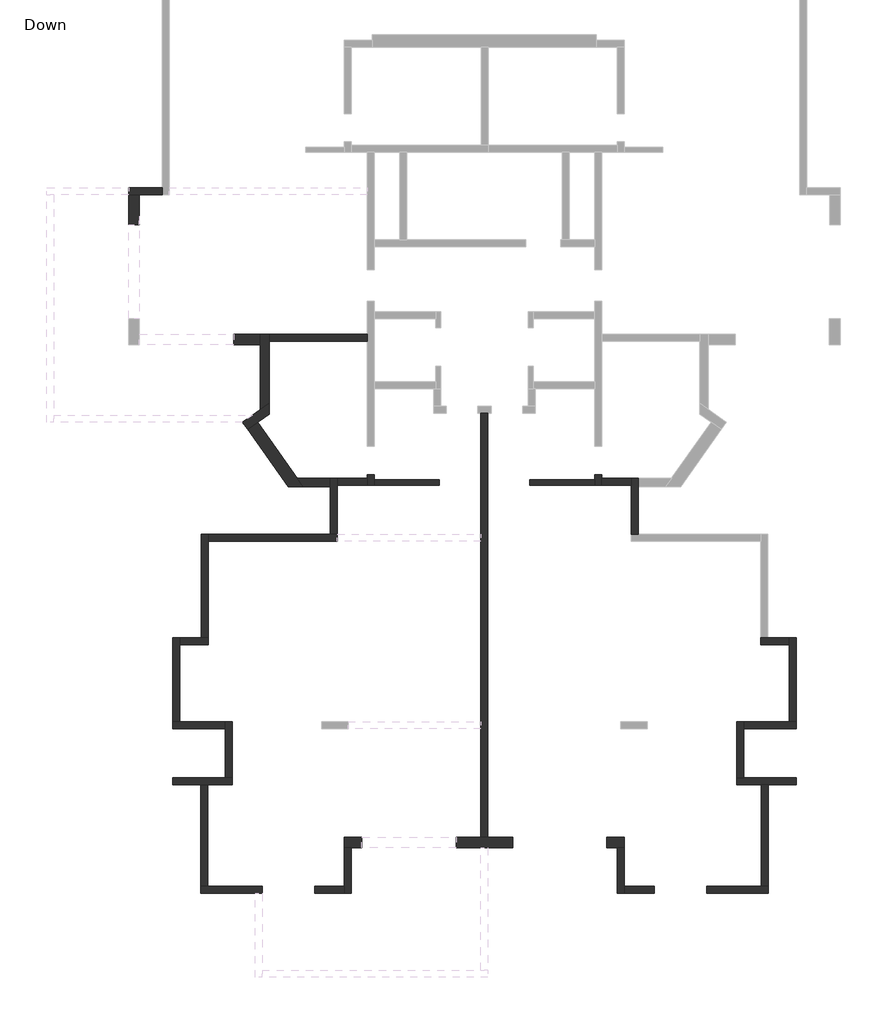
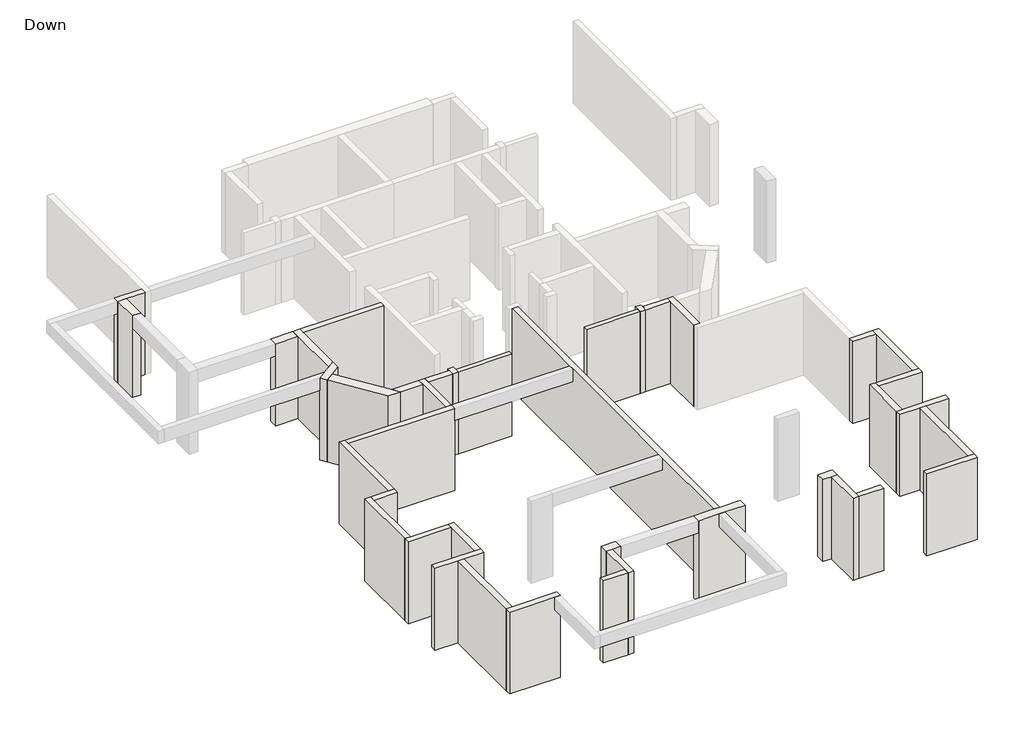
# One storey, part 1 of 3: 40 walls.
"""IFC4 building model written with IfcOpenShell, lengths in millimetres."""

import ifcopenshell
import ifcopenshell.guid

model = None  # the IFC model being written
_history = None  # IfcOwnerHistory: only IFC2X3 demands one
_inside = {}  # id of a spatial element -> (the spatial element, [elements in it])
_under = {}  # id of a project, library or spatial element -> (it, [spatial elements below it])
_declared = {}  # id of a project -> (the project, [libraries it declares])
_typed = {}  # id of a type object -> (the type object, [elements of that type])
_made_of = {}  # id of a material, layer set ... -> (it, [elements and type objects made of it])


def new_model(schema):
    """Start an empty IFC model of exactly this schema.

    Asked for "IFC4X3", IfcOpenShell would pick the latest addendum, in which some entities
    have other attributes; the version numbers below select the first issue.
    IFC2X3 requires an IfcOwnerHistory on every rooted entity: one is made here for all.
    """
    global model, _history
    if schema == "IFC4X3":
        model = ifcopenshell.file(schema_version=(4, 3, 0, 0))
    else:
        model = ifcopenshell.file(schema=schema)
    _inside.clear()
    _under.clear()
    _declared.clear()
    _typed.clear()
    _made_of.clear()
    _history = None
    if model.schema == "IFC2X3":
        org = make("IfcOrganization", Name="unknown")
        user = make(
            "IfcPersonAndOrganization",
            ThePerson=make("IfcPerson", FamilyName="unknown"),
            TheOrganization=org,
        )
        app = make(
            "IfcApplication",
            ApplicationDeveloper=org,
            Version="unknown",
            ApplicationFullName="unknown",
            ApplicationIdentifier="unknown",
        )
        _history = make(
            "IfcOwnerHistory",
            OwningUser=user,
            OwningApplication=app,
            ChangeAction="ADDED",
            CreationDate=0,
        )
    return model


def make(cls, **values):
    """One entity of the class cls with the attributes given. An attribute that is None is left unset."""
    return model.create_entity(
        cls, **{name: value for name, value in values.items() if value is not None}
    )


def rooted(cls, **values):
    """An entity with a GlobalId (a new one), such as an element, a storey or a relation."""
    return make(cls, GlobalId=ifcopenshell.guid.new(), OwnerHistory=_history, **values)


def si_unit(unit_type, name, prefix=None):
    """IfcSIUnit, for example si_unit("LENGTHUNIT", "METRE", prefix="MILLI")."""
    return make("IfcSIUnit", UnitType=unit_type, Prefix=prefix, Name=name)


def assignment(units):
    """IfcUnitAssignment: the units of a project."""
    return None if units is None else make("IfcUnitAssignment", Units=units)


def point(xyz):
    """IfcCartesianPoint."""
    return None if xyz is None else make("IfcCartesianPoint", Coordinates=xyz)


def direction(xyz):
    """IfcDirection."""
    return None if xyz is None else make("IfcDirection", DirectionRatios=xyz)


def frame(location, z_axis=None, x_axis=None):
    """IfcAxis2Placement3D, a coordinate frame: its origin and axes. An axis left out is left unset."""
    return make(
        "IfcAxis2Placement3D",
        Location=point(location),
        Axis=direction(z_axis),
        RefDirection=direction(x_axis),
    )


def origin():
    """The frame at (0, 0, 0) with its axes left unset."""
    return frame((0.0, 0.0, 0.0))


def place(relative_to, where):
    """IfcLocalPlacement: puts the frame where relative to a parent placement (None: the world)."""
    return make(
        "IfcLocalPlacement", PlacementRelTo=relative_to, RelativePlacement=where
    )


def context(
    kind, dimensions, precision=None, world=None, true_north=None, identifier=None
):
    """IfcGeometricRepresentationContext, for example the 3D "Model" context."""
    return make(
        "IfcGeometricRepresentationContext",
        ContextIdentifier=identifier,
        ContextType=kind,
        CoordinateSpaceDimension=dimensions,
        Precision=precision,
        WorldCoordinateSystem=world,
        TrueNorth=true_north,
    )


def project(units=None, contexts=None):
    """IfcProject with its units and contexts."""
    return rooted(
        "IfcProject",
        Name="project",
        RepresentationContexts=contexts,
        UnitsInContext=assignment(units),
    )


def spatial(cls, under=None, at=None, **own):
    """A site, building, storey or space (cls), placed at a placement, below another one or the project."""
    s = rooted(cls, ObjectPlacement=at, **own)
    if under is not None:
        _under.setdefault(under.id(), (under, []))[1].append(s)
    return s


def faces_of(points, faces, orient=None, outer=None):
    """IfcFace entities. A face is a list of loops; a loop is a list of indices into points, from 0.

    orient and outer hold one flag for each loop. By default every Orientation is true, the
    first loop of a face is its IfcFaceOuterBound and the others are IfcFaceBound.
    """
    made = []
    for i, loops in enumerate(faces):
        bounds = []
        for j, loop in enumerate(loops):
            is_outer = j == 0 if outer is None else outer[i][j]
            bounds.append(
                make(
                    "IfcFaceOuterBound" if is_outer else "IfcFaceBound",
                    Bound=make("IfcPolyLoop", Polygon=[points[k] for k in loop]),
                    Orientation=True if orient is None else orient[i][j],
                )
            )
        made.append(make("IfcFace", Bounds=bounds))
    return made


def faceted_brep(points, faces, orient=None, outer=None, voids=None):
    """IfcFacetedBrep: a solid bounded by flat faces; with voids (closed shells), ...WithVoids."""
    shared = [point(p) for p in points]
    hull = make("IfcClosedShell", CfsFaces=faces_of(shared, faces, orient, outer))
    if voids is None:
        return make("IfcFacetedBrep", Outer=hull)
    return make(
        "IfcFacetedBrepWithVoids",
        Outer=hull,
        Voids=[
            make(cls, CfsFaces=faces_of(shared, fs, o, b)) for cls, fs, o, b in voids
        ],
    )


def shape(context_of_items, identifier, shape_type, items):
    """IfcShapeRepresentation: the items that make up one representation, for example the "Body"."""
    return make(
        "IfcShapeRepresentation",
        ContextOfItems=context_of_items,
        RepresentationIdentifier=identifier,
        RepresentationType=shape_type,
        Items=items,
    )


def made_of(thing, what):
    """Note that an element or type object is made of a material, layer set ...; save() writes the relation."""
    if what is not None:
        _made_of.setdefault(what.id(), (what, []))[1].append(thing)
    return thing


def element(
    cls,
    number,
    at=None,
    inside=None,
    cuts=None,
    type_object=None,
    material=None,
    context=None,
    identifier="Body",
    shape_type=None,
    held_by="IfcProductDefinitionShape",
    body=None,
    shapes=None,
    **own,
):
    """One element of the class cls, such as IfcWall. Its Tag is "e" and its number.

    at: its placement. inside: the storey or other place that contains it. cuts: it is an
    opening in that element (IfcRelVoidsElement). A single representation is given by context,
    identifier, shape_type and body (its items); several are given by shapes. held_by: the class
    of the entity that holds the representations. save() writes the other relations.
    """
    e = rooted(cls, Tag="e%d" % number, ObjectPlacement=at, **own)
    if body is not None:
        shapes = [shape(context, identifier, shape_type, body)]
    if shapes is not None:
        e.Representation = make(held_by, Representations=shapes)
    if inside is not None:
        _inside.setdefault(inside.id(), (inside, []))[1].append(e)
    if cuts is not None:
        rooted(
            "IfcRelVoidsElement", RelatingBuildingElement=cuts, RelatedOpeningElement=e
        )
    if type_object is not None:
        _typed.setdefault(type_object.id(), (type_object, []))[1].append(e)
    return made_of(e, material)


def aggregate(whole, parts):
    """IfcRelAggregates: a whole, such as a stair, and the parts it consists of."""
    return rooted("IfcRelAggregates", RelatingObject=whole, RelatedObjects=parts)


def save(model, path):
    """Write the relations noted so far, then the file.

    IfcRelAggregates (storeys below a building ...), IfcRelContainedInSpatialStructure (elements
    in a storey), IfcRelDefinesByType, IfcRelAssociatesMaterial and IfcRelDeclares: one each for
    every whole, place, type object, material and project.
    """
    for whole, parts in _under.values():
        aggregate(whole, parts)
    for where, things in _inside.values():
        rooted(
            "IfcRelContainedInSpatialStructure",
            RelatedElements=things,
            RelatingStructure=where,
        )
    for kind, things in _typed.values():
        rooted("IfcRelDefinesByType", RelatedObjects=things, RelatingType=kind)
    for what, things in _made_of.values():
        rooted("IfcRelAssociatesMaterial", RelatedObjects=things, RelatingMaterial=what)
    for by, libraries in _declared.values():
        rooted("IfcRelDeclares", RelatingContext=by, RelatedDefinitions=libraries)
    model.write(path)


model = new_model("IFC4")

# Units and contexts
model_context = context("Model", 3, world=origin())
ifc_project = project(units=[si_unit("LENGTHUNIT", "METRE", prefix="MILLI")], contexts=[model_context])

# Site, building, storey
site = spatial("IfcSite", under=ifc_project)
building = spatial("IfcBuilding", under=site)
storey = spatial("IfcBuildingStorey", under=building, Name="Down", Elevation=0.0)

# Walls
placement = place(None, origin())
element("IfcWall", 1, ObjectType="15", at=placement, inside=storey, context=model_context, shape_type="Brep", body=[
    faceted_brep([(877.2376347, -8447.6409767, 0.0), (2726.9065089, -8447.6409767, 0.0), (2726.9065089, -8447.6409767, 2800.0), (2726.9065089, -8447.6409767, 3000.0), (877.2376347, -8447.6409767, 3000.0), (877.2376347, -8297.6409767, 0.0), (877.2376347, -8297.6409767, 2800.0), (877.2376347, -8297.6409767, 3000.0), (2726.9065089, -8297.6409767, 3000.0), (2726.9065089, -8297.6409767, 2800.0), (2726.9065089, -8297.6409767, 0.0)], [[[0, 1, 2, 3, 4]], [[5, 6, 7, 8, 9, 10]], [[1, 0, 5, 10]], [[3, 2, 1, 10, 9, 8]], [[4, 3, 8, 7]], [[0, 4, 7, 6, 5]]]),
])
element("IfcWall", 2, ObjectType="15", at=placement, inside=storey, context=model_context, shape_type="Brep", body=[
    faceted_brep([(7169.9528665, -8297.6409767, 0.0), (5320.2839923, -8297.6409767, 0.0), (5320.2839923, -8297.6409767, 2800.0), (5320.2839923, -8297.6409767, 3000.0), (7169.9528665, -8297.6409767, 3000.0), (7169.9528665, -8297.6409767, 2800.0), (7169.9528665, -8447.6409767, 0.0), (7169.9528665, -8447.6409767, 3000.0), (5320.2839923, -8447.6409767, 3000.0), (5320.2839923, -8447.6409767, 2800.0), (5320.2839923, -8447.6409767, 0.0)], [[[0, 1, 2, 3, 4, 5]], [[6, 7, 8, 9, 10]], [[1, 0, 6, 10]], [[3, 2, 1, 10, 9, 8]], [[4, 3, 8, 7]], [[0, 5, 4, 7, 6]]]),
])
element("IfcWall", 3, ObjectType="20", at=placement, inside=storey, context=model_context, shape_type="Brep", body=[
    faceted_brep([(-5177.0670011, 46.6636591, 0.0), (-6127.9594861, 46.6636591, 0.0), (-6127.9594861, 46.6636591, 2550.0), (-6127.9594861, 46.6636591, 3000.0), (-5177.0670011, 46.6636591, 3000.0), (-5177.0670011, -153.3363409, 0.0), (-5177.0670011, -153.3363409, 3000.0), (-5827.9594861, -153.3363409, 3000.0), (-6127.9594861, -153.3363409, 3000.0), (-6127.9594861, -153.3363409, 2550.0), (-6127.9594861, -153.3363409, 0.0), (-5827.9594861, -153.3363409, 0.0)], [[[0, 1, 2, 3, 4]], [[5, 6, 7, 8, 9, 10, 11]], [[1, 0, 5, 11, 10]], [[4, 3, 8, 7, 6]], [[0, 4, 6, 5]], [[3, 2, 1, 10, 9, 8]]]),
])
element("IfcWall", 4, ObjectType="20", at=placement, inside=storey, context=model_context, shape_type="Brep", body=[
    faceted_brep([(3923.5952506, -6391.6807118, 0.0), (3923.5952506, -18496.3164734, 0.0), (3923.5952506, -18496.3164734, 2800.0), (3923.5952506, -18496.3164734, 3000.0), (3923.5952506, -15399.2157792, 3000.0), (3923.5952506, -15199.2157792, 3000.0), (3923.5952506, -10045.6542217, 3000.0), (3923.5952506, -9845.6542217, 3000.0), (3923.5952506, -6391.6807118, 3000.0), (3923.5952506, -6391.6807118, 2800.0), (4123.5952506, -6391.6807118, 0.0), (4123.5952506, -6391.6807118, 2800.0), (4123.5952506, -6391.6807118, 3000.0), (4123.5952506, -9845.6542217, 3000.0), (4123.5952506, -10045.6542217, 3000.0), (4123.5952506, -15199.2157792, 3000.0), (4123.5952506, -15399.2157792, 3000.0), (4123.5952506, -18496.3164734, 3000.0), (4123.5952506, -18496.3164734, 2800.0), (4123.5952506, -18496.3164734, 0.0)], [[[0, 1, 2, 3, 4, 5, 6, 7, 8, 9]], [[10, 11, 12, 13, 14, 15, 16, 17, 18, 19]], [[1, 0, 10, 19]], [[8, 7, 6, 5, 4, 3, 17, 16, 15, 14, 13, 12]], [[0, 9, 8, 12, 11, 10]], [[3, 2, 1, 19, 18, 17]]]),
])
element("IfcWall", 5, ObjectType="20", at=placement, inside=storey, context=model_context, shape_type="Brep", body=[
    faceted_brep([(27.8998864, -18796.3164734, 0.0), (27.8998864, -19900.6211091, 0.0), (27.8998864, -20100.6211091, 0.0), (27.8998864, -20100.6211091, 3000.0), (27.8998864, -19900.6211091, 3000.0), (27.8998864, -18796.3164734, 3000.0), (227.8998864, -18796.3164734, 0.0), (227.8998864, -18796.3164734, 2800.0), (227.8998864, -18796.3164734, 3000.0), (227.8998864, -20100.6211091, 3000.0), (227.8998864, -20100.6211091, 2800.0), (227.8998864, -20100.6211091, 0.0)], [[[0, 1, 2, 3, 4, 5]], [[6, 7, 8, 9, 10, 11]], [[2, 1, 0, 6, 11]], [[5, 4, 3, 9, 8]], [[0, 5, 8, 7, 6]], [[3, 2, 11, 10, 9]]]),
])
element("IfcWall", 6, ObjectType="20", at=placement, inside=storey, context=model_context, shape_type="Brep", body=[
    faceted_brep([(27.8998864, -19900.6211091, 0.0), (-827.7292527, -19900.6211091, 0.0), (-827.7292527, -19900.6211091, 2800.0), (-827.7292527, -19900.6211091, 3000.0), (27.8998864, -19900.6211091, 3000.0), (27.8998864, -19900.6211091, 2800.0), (27.8998864, -20100.6211091, 0.0), (27.8998864, -20100.6211091, 3000.0), (-827.7292527, -20100.6211091, 3000.0), (-827.7292527, -20100.6211091, 2800.0), (-827.7292527, -20100.6211091, 0.0)], [[[0, 1, 2, 3, 4, 5]], [[6, 7, 8, 9, 10]], [[1, 0, 6, 10]], [[3, 2, 1, 10, 9, 8]], [[4, 3, 8, 7]], [[0, 5, 4, 7, 6]]]),
])
element("IfcWall", 7, ObjectType="20", at=placement, inside=storey, context=model_context, shape_type="Brep", body=[
    faceted_brep([(-2325.0802461, -19900.6211091, 0.0), (-3874.0868686, -19900.6211091, 0.0), (-4074.0868686, -19900.6211091, 0.0), (-4074.0868686, -19900.6211091, 3000.0), (-3874.0868686, -19900.6211091, 3000.0), (-2325.0802461, -19900.6211091, 3000.0), (-2325.0802461, -19900.6211091, 2800.0), (-2325.0802461, -20100.6211091, 0.0), (-2325.0802461, -20100.6211091, 2800.0), (-2325.0802461, -20100.6211091, 3000.0), (-4074.0868686, -20100.6211091, 3000.0), (-4074.0868686, -20100.6211091, 0.0)], [[[0, 1, 2, 3, 4, 5, 6]], [[7, 8, 9, 10, 11]], [[2, 1, 0, 7, 11]], [[5, 4, 3, 10, 9]], [[0, 6, 5, 9, 8, 7]], [[3, 2, 11, 10]]]),
])
element("IfcWall", 8, ObjectType="20", at=placement, inside=storey, context=model_context, shape_type="Brep", body=[
    faceted_brep([(-3874.0868686, -19900.6211091, 0.0), (-3874.0868686, -16998.96548, 0.0), (-3874.0868686, -16998.96548, 2800.0), (-3874.0868686, -16998.96548, 3000.0), (-3874.0868686, -19900.6211091, 3000.0), (-3874.0868686, -19900.6211091, 2800.0), (-4074.0868686, -19900.6211091, 0.0), (-4074.0868686, -19900.6211091, 3000.0), (-4074.0868686, -16998.96548, 3000.0), (-4074.0868686, -16998.96548, 0.0)], [[[0, 1, 2, 3, 4, 5]], [[6, 7, 8, 9]], [[1, 0, 6, 9]], [[4, 3, 8, 7]], [[0, 5, 4, 7, 6]], [[3, 2, 1, 9, 8]]]),
])
element("IfcWall", 9, ObjectType="20", at=placement, inside=storey, context=model_context, shape_type="Brep", body=[
    faceted_brep([(-4873.0934911, -16998.96548, 0.0), (-4074.0868686, -16998.96548, 0.0), (-3874.0868686, -16998.96548, 0.0), (-3174.4179944, -16998.96548, 0.0), (-3174.4179944, -16998.96548, 2800.0), (-3174.4179944, -16998.96548, 3000.0), (-3874.0868686, -16998.96548, 3000.0), (-4074.0868686, -16998.96548, 3000.0), (-4873.0934911, -16998.96548, 3000.0), (-4873.0934911, -16798.96548, 0.0), (-4873.0934911, -16798.96548, 3000.0), (-3374.4179944, -16798.96548, 3000.0), (-3174.4179944, -16798.96548, 3000.0), (-3174.4179944, -16798.96548, 0.0), (-3374.4179944, -16798.96548, 0.0)], [[[0, 1, 2, 3, 4, 5, 6, 7, 8]], [[9, 10, 11, 12, 13, 14]], [[3, 2, 1, 0, 9, 14, 13]], [[8, 7, 6, 5, 12, 11, 10]], [[0, 8, 10, 9]], [[5, 4, 3, 13, 12]]]),
])
element("IfcWall", 10, ObjectType="20", at=placement, inside=storey, context=model_context, shape_type="Brep", body=[
    faceted_brep([(-3174.4179944, -16798.96548, 0.0), (-3174.4179944, -15196.978725, 0.0), (-3174.4179944, -15196.978725, 2800.0), (-3174.4179944, -15196.978725, 3000.0), (-3174.4179944, -16798.96548, 3000.0), (-3374.4179944, -16798.96548, 0.0), (-3374.4179944, -16798.96548, 3000.0), (-3374.4179944, -15396.978725, 3000.0), (-3374.4179944, -15196.978725, 3000.0), (-3374.4179944, -15196.978725, 0.0), (-3374.4179944, -15396.978725, 0.0)], [[[0, 1, 2, 3, 4]], [[5, 6, 7, 8, 9, 10]], [[1, 0, 5, 10, 9]], [[4, 3, 8, 7, 6]], [[0, 4, 6, 5]], [[3, 2, 1, 9, 8]]]),
])
element("IfcWall", 11, ObjectType="20", at=placement, inside=storey, context=model_context, shape_type="Brep", body=[
    faceted_brep([(-4673.0934911, -15196.978725, 0.0), (-4673.0934911, -12996.3164734, 0.0), (-4673.0934911, -12796.3164734, 0.0), (-4673.0934911, -12796.3164734, 3000.0), (-4673.0934911, -12996.3164734, 3000.0), (-4673.0934911, -15196.978725, 3000.0), (-4673.0934911, -15196.978725, 2800.0), (-4873.0934911, -15196.978725, 0.0), (-4873.0934911, -15196.978725, 3000.0), (-4873.0934911, -12796.3164734, 3000.0), (-4873.0934911, -12796.3164734, 0.0)], [[[0, 1, 2, 3, 4, 5, 6]], [[7, 8, 9, 10]], [[2, 1, 0, 7, 10]], [[5, 4, 3, 9, 8]], [[3, 2, 10, 9]], [[0, 6, 5, 8, 7]]]),
])
element("IfcWall", 12, ObjectType="20", at=placement, inside=storey, context=model_context, shape_type="Brep", body=[
    faceted_brep([(-4673.0934911, -12996.3164734, 0.0), (-3860.1795838, -12996.3164734, 0.0), (-3860.1795838, -12996.3164734, 2800.0), (-3860.1795838, -12996.3164734, 3000.0), (-4673.0934911, -12996.3164734, 3000.0), (-4673.0934911, -12996.3164734, 2800.0), (-4673.0934911, -12796.3164734, 0.0), (-4673.0934911, -12796.3164734, 3000.0), (-4060.1795838, -12796.3164734, 3000.0), (-3860.1795838, -12796.3164734, 3000.0), (-3860.1795838, -12796.3164734, 0.0), (-4060.1795838, -12796.3164734, 0.0)], [[[0, 1, 2, 3, 4, 5]], [[6, 7, 8, 9, 10, 11]], [[1, 0, 6, 11, 10]], [[4, 3, 9, 8, 7]], [[0, 5, 4, 7, 6]], [[3, 2, 1, 10, 9]]]),
])
element("IfcWall", 13, ObjectType="20", at=placement, inside=storey, context=model_context, shape_type="Brep", body=[
    faceted_brep([(-3860.1795838, -12796.3164734, 0.0), (-3860.1795838, -10045.6542217, 0.0), (-3860.1795838, -9845.6542217, 0.0), (-3860.1795838, -9845.6542217, 3000.0), (-3860.1795838, -10045.6542217, 3000.0), (-3860.1795838, -12796.3164734, 3000.0), (-4060.1795838, -12796.3164734, 0.0), (-4060.1795838, -12796.3164734, 3000.0), (-4060.1795838, -9845.6542217, 3000.0), (-4060.1795838, -9845.6542217, 0.0)], [[[0, 1, 2, 3, 4, 5]], [[6, 7, 8, 9]], [[2, 1, 0, 6, 9]], [[5, 4, 3, 8, 7]], [[0, 5, 7, 6]], [[3, 2, 9, 8]]]),
])
element("IfcWall", 14, ObjectType="20", at=placement, inside=storey, context=model_context, shape_type="Brep", body=[
    faceted_brep([(-3860.1795838, -10045.6542217, 0.0), (-173.424617, -10045.6542217, 0.0), (-173.424617, -10045.6542217, 2550.0), (-173.424617, -10045.6542217, 3000.0), (-3860.1795838, -10045.6542217, 3000.0), (-3860.1795838, -10045.6542217, 2800.0), (-3860.1795838, -9845.6542217, 0.0), (-3860.1795838, -9845.6542217, 3000.0), (-373.424617, -9845.6542217, 3000.0), (-173.424617, -9845.6542217, 3000.0), (-173.424617, -9845.6542217, 2550.0), (-173.424617, -9845.6542217, 0.0), (-373.424617, -9845.6542217, 0.0)], [[[0, 1, 2, 3, 4, 5]], [[6, 7, 8, 9, 10, 11, 12]], [[1, 0, 6, 12, 11]], [[4, 3, 9, 8, 7]], [[0, 5, 4, 7, 6]], [[3, 2, 1, 11, 10, 9]]]),
])
element("IfcWall", 15, ObjectType="20", at=placement, inside=storey, context=model_context, shape_type="Brep", body=[
    faceted_brep([(-173.424617, -9845.6542217, 0.0), (-173.424617, -8447.6409767, 0.0), (-173.424617, -8247.6409767, 0.0), (-173.424617, -8247.6409767, 3000.0), (-173.424617, -8447.6409767, 3000.0), (-173.424617, -9845.6542217, 3000.0), (-173.424617, -9845.6542217, 2800.0), (-373.424617, -9845.6542217, 0.0), (-373.424617, -9845.6542217, 3000.0), (-373.424617, -8497.6409767, 3000.0), (-373.424617, -8247.6409767, 3000.0), (-373.424617, -8247.6409767, 0.0), (-373.424617, -8497.6409767, 0.0)], [[[0, 1, 2, 3, 4, 5, 6]], [[7, 8, 9, 10, 11, 12]], [[2, 1, 0, 7, 12, 11]], [[5, 4, 3, 10, 9, 8]], [[0, 6, 5, 8, 7]], [[3, 2, 11, 10]]]),
])
element("IfcWall", 16, ObjectType="20", at=placement, inside=storey, context=model_context, shape_type="Brep", body=[
    faceted_brep([(-173.424617, -8447.6409767, 0.0), (677.2376347, -8447.6409767, 0.0), (677.2376347, -8447.6409767, 3000.0), (-173.424617, -8447.6409767, 3000.0), (-173.424617, -8447.6409767, 2800.0), (-173.424617, -8247.6409767, 0.0), (-173.424617, -8247.6409767, 3000.0), (677.2376347, -8247.6409767, 3000.0), (677.2376347, -8247.6409767, 2800.0), (677.2376347, -8247.6409767, 0.0)], [[[0, 1, 2, 3, 4]], [[5, 6, 7, 8, 9]], [[1, 0, 5, 9]], [[3, 2, 7, 6]], [[0, 4, 3, 6, 5]], [[2, 1, 9, 8, 7]]]),
])
element("IfcWall", 17, ObjectType="20", at=placement, inside=storey, context=model_context, shape_type="Brep", body=[
    faceted_brep([(-2120.7912039, -4340.6873343, 0.0), (675.9131314, -4340.6873343, 0.0), (675.9131314, -4340.6873343, 2800.0), (675.9131314, -4340.6873343, 3000.0), (-2120.7912039, -4340.6873343, 3000.0), (-2120.7912039, -4340.6873343, 2800.0), (-2120.7912039, -4140.6873343, 0.0), (-2120.7912039, -4140.6873343, 3000.0), (675.9131314, -4140.6873343, 3000.0), (675.9131314, -4140.6873343, 2800.0), (675.9131314, -4140.6873343, 0.0)], [[[0, 1, 2, 3, 4, 5]], [[6, 7, 8, 9, 10]], [[1, 0, 6, 10]], [[4, 3, 8, 7]], [[0, 5, 4, 7, 6]], [[3, 2, 1, 10, 9, 8]]]),
])
element("IfcWall", 18, ObjectType="20", at=placement, inside=storey, context=model_context, shape_type="Brep", body=[
    faceted_brep([(-4873.0934911, -15396.978725, 0.0), (-3374.4179944, -15396.978725, 0.0), (-3374.4179944, -15396.978725, 3000.0), (-4873.0934911, -15396.978725, 3000.0), (-4873.0934911, -15196.978725, 0.0), (-4873.0934911, -15196.978725, 3000.0), (-4673.0934911, -15196.978725, 3000.0), (-3374.4179944, -15196.978725, 3000.0), (-3374.4179944, -15196.978725, 0.0), (-4673.0934911, -15196.978725, 0.0)], [[[0, 1, 2, 3]], [[4, 5, 6, 7, 8, 9]], [[1, 0, 4, 9, 8]], [[3, 2, 7, 6, 5]], [[2, 1, 8, 7]], [[0, 3, 5, 4]]]),
])
element("IfcWall", 19, ObjectType="20", at=placement, inside=storey, context=model_context, shape_type="Brep", body=[
    faceted_brep([(677.2376347, -8146.978725, 0.0), (677.2376347, -8247.6409767, 0.0), (677.2376347, -8447.6409767, 0.0), (677.2376347, -8447.6409767, 3000.0), (677.2376347, -8247.6409767, 3000.0), (677.2376347, -8146.978725, 3000.0), (677.2376347, -8146.978725, 2800.0), (877.2376347, -8146.978725, 0.0), (877.2376347, -8146.978725, 2800.0), (877.2376347, -8146.978725, 3000.0), (877.2376347, -8297.6409767, 3000.0), (877.2376347, -8447.6409767, 3000.0), (877.2376347, -8447.6409767, 0.0), (877.2376347, -8297.6409767, 0.0)], [[[0, 1, 2, 3, 4, 5, 6]], [[7, 8, 9, 10, 11, 12, 13]], [[2, 1, 0, 7, 13, 12]], [[5, 4, 3, 11, 10, 9]], [[0, 6, 5, 9, 8, 7]], [[3, 2, 12, 11]]]),
])
element("IfcWall", 20, ObjectType="20", at=placement, inside=storey, context=model_context, shape_type="Brep", body=[
    faceted_brep([(7819.2906148, -18796.3164734, 0.0), (7819.2906148, -20100.6211091, 0.0), (7819.2906148, -20100.6211091, 2800.0), (7819.2906148, -20100.6211091, 3000.0), (7819.2906148, -18796.3164734, 3000.0), (7819.2906148, -18796.3164734, 2800.0), (8019.2906148, -18796.3164734, 0.0), (8019.2906148, -18796.3164734, 3000.0), (8019.2906148, -19900.6211091, 3000.0), (8019.2906148, -20100.6211091, 3000.0), (8019.2906148, -20100.6211091, 0.0), (8019.2906148, -19900.6211091, 0.0)], [[[0, 1, 2, 3, 4, 5]], [[6, 7, 8, 9, 10, 11]], [[1, 0, 6, 11, 10]], [[4, 3, 9, 8, 7]], [[0, 5, 4, 7, 6]], [[3, 2, 1, 10, 9]]]),
])
element("IfcWall", 21, ObjectType="20", at=placement, inside=storey, context=model_context, shape_type="Brep", body=[
    faceted_brep([(8019.2906148, -20100.6211091, 0.0), (8874.9197539, -20100.6211091, 0.0), (8874.9197539, -20100.6211091, 2800.0), (8874.9197539, -20100.6211091, 3000.0), (8019.2906148, -20100.6211091, 3000.0), (8019.2906148, -19900.6211091, 0.0), (8019.2906148, -19900.6211091, 2800.0), (8019.2906148, -19900.6211091, 3000.0), (8874.9197539, -19900.6211091, 3000.0), (8874.9197539, -19900.6211091, 2800.0), (8874.9197539, -19900.6211091, 0.0)], [[[0, 1, 2, 3, 4]], [[5, 6, 7, 8, 9, 10]], [[1, 0, 5, 10]], [[3, 2, 1, 10, 9, 8]], [[4, 3, 8, 7]], [[0, 4, 7, 6, 5]]]),
])
element("IfcWall", 22, ObjectType="20", at=placement, inside=storey, context=model_context, shape_type="Brep", body=[
    faceted_brep([(10372.2707473, -20100.6211091, 0.0), (12121.2773698, -20100.6211091, 0.0), (12121.2773698, -20100.6211091, 3000.0), (10372.2707473, -20100.6211091, 3000.0), (10372.2707473, -20100.6211091, 2800.0), (10372.2707473, -19900.6211091, 0.0), (10372.2707473, -19900.6211091, 2800.0), (10372.2707473, -19900.6211091, 3000.0), (11921.2773698, -19900.6211091, 3000.0), (12121.2773698, -19900.6211091, 3000.0), (12121.2773698, -19900.6211091, 0.0), (11921.2773698, -19900.6211091, 0.0)], [[[0, 1, 2, 3, 4]], [[5, 6, 7, 8, 9, 10, 11]], [[1, 0, 5, 11, 10]], [[3, 2, 9, 8, 7]], [[0, 4, 3, 7, 6, 5]], [[2, 1, 10, 9]]]),
])
element("IfcWall", 23, ObjectType="20", at=placement, inside=storey, context=model_context, shape_type="Brep", body=[
    faceted_brep([(12121.2773698, -19900.6211091, 0.0), (12121.2773698, -16998.96548, 0.0), (12121.2773698, -16998.96548, 3000.0), (12121.2773698, -19900.6211091, 3000.0), (11921.2773698, -19900.6211091, 0.0), (11921.2773698, -19900.6211091, 2800.0), (11921.2773698, -19900.6211091, 3000.0), (11921.2773698, -16998.96548, 3000.0), (11921.2773698, -16998.96548, 2800.0), (11921.2773698, -16998.96548, 0.0)], [[[0, 1, 2, 3]], [[4, 5, 6, 7, 8, 9]], [[1, 0, 4, 9]], [[3, 2, 7, 6]], [[0, 3, 6, 5, 4]], [[2, 1, 9, 8, 7]]]),
])
element("IfcWall", 24, ObjectType="20", at=placement, inside=storey, context=model_context, shape_type="Brep", body=[
    faceted_brep([(12920.2839923, -16798.96548, 0.0), (11421.6084956, -16798.96548, 0.0), (11221.6084956, -16798.96548, 0.0), (11221.6084956, -16798.96548, 3000.0), (11421.6084956, -16798.96548, 3000.0), (12920.2839923, -16798.96548, 3000.0), (12920.2839923, -16998.96548, 0.0), (12920.2839923, -16998.96548, 3000.0), (12121.2773698, -16998.96548, 3000.0), (11921.2773698, -16998.96548, 3000.0), (11221.6084956, -16998.96548, 3000.0), (11221.6084956, -16998.96548, 2800.0), (11221.6084956, -16998.96548, 0.0), (11921.2773698, -16998.96548, 0.0), (12121.2773698, -16998.96548, 0.0)], [[[0, 1, 2, 3, 4, 5]], [[6, 7, 8, 9, 10, 11, 12, 13, 14]], [[2, 1, 0, 6, 14, 13, 12]], [[5, 4, 3, 10, 9, 8, 7]], [[0, 5, 7, 6]], [[3, 2, 12, 11, 10]]]),
])
element("IfcWall", 25, ObjectType="20", at=placement, inside=storey, context=model_context, shape_type="Brep", body=[
    faceted_brep([(11421.6084956, -16798.96548, 0.0), (11421.6084956, -15396.978725, 0.0), (11421.6084956, -15196.978725, 0.0), (11421.6084956, -15196.978725, 3000.0), (11421.6084956, -15396.978725, 3000.0), (11421.6084956, -16798.96548, 3000.0), (11221.6084956, -16798.96548, 0.0), (11221.6084956, -16798.96548, 3000.0), (11221.6084956, -15196.978725, 3000.0), (11221.6084956, -15196.978725, 2800.0), (11221.6084956, -15196.978725, 0.0)], [[[0, 1, 2, 3, 4, 5]], [[6, 7, 8, 9, 10]], [[2, 1, 0, 6, 10]], [[5, 4, 3, 8, 7]], [[0, 5, 7, 6]], [[3, 2, 10, 9, 8]]]),
])
element("IfcWall", 26, ObjectType="20", at=placement, inside=storey, context=model_context, shape_type="Brep", body=[
    faceted_brep([(12920.2839923, -15196.978725, 0.0), (12920.2839923, -12796.3164734, 0.0), (12920.2839923, -12796.3164734, 3000.0), (12920.2839923, -15196.978725, 3000.0), (12720.2839923, -15196.978725, 0.0), (12720.2839923, -15196.978725, 2800.0), (12720.2839923, -15196.978725, 3000.0), (12720.2839923, -12996.3164734, 3000.0), (12720.2839923, -12796.3164734, 3000.0), (12720.2839923, -12796.3164734, 0.0), (12720.2839923, -12996.3164734, 0.0)], [[[0, 1, 2, 3]], [[4, 5, 6, 7, 8, 9, 10]], [[1, 0, 4, 10, 9]], [[3, 2, 8, 7, 6]], [[2, 1, 9, 8]], [[0, 3, 6, 5, 4]]]),
])
element("IfcWall", 27, ObjectType="20", at=placement, inside=storey, context=model_context, shape_type="Brep", body=[
    faceted_brep([(12720.2839923, -12796.3164734, 0.0), (12107.370085, -12796.3164734, 0.0), (11907.370085, -12796.3164734, 0.0), (11907.370085, -12796.3164734, 3000.0), (12107.370085, -12796.3164734, 3000.0), (12720.2839923, -12796.3164734, 3000.0), (12720.2839923, -12996.3164734, 0.0), (12720.2839923, -12996.3164734, 2800.0), (12720.2839923, -12996.3164734, 3000.0), (11907.370085, -12996.3164734, 3000.0), (11907.370085, -12996.3164734, 2800.0), (11907.370085, -12996.3164734, 0.0)], [[[0, 1, 2, 3, 4, 5]], [[6, 7, 8, 9, 10, 11]], [[2, 1, 0, 6, 11]], [[5, 4, 3, 9, 8]], [[0, 5, 8, 7, 6]], [[3, 2, 11, 10, 9]]]),
])
element("IfcWall", 28, ObjectType="20", at=placement, inside=storey, context=model_context, shape_type="Brep", body=[
    faceted_brep([(8420.6151181, -9845.6542217, 0.0), (8420.6151181, -8497.6409767, 0.0), (8420.6151181, -8247.6409767, 0.0), (8420.6151181, -8247.6409767, 3000.0), (8420.6151181, -8497.6409767, 3000.0), (8420.6151181, -9845.6542217, 3000.0), (8220.6151181, -9845.6542217, 0.0), (8220.6151181, -9845.6542217, 2800.0), (8220.6151181, -9845.6542217, 3000.0), (8220.6151181, -8447.6409767, 3000.0), (8220.6151181, -8247.6409767, 3000.0), (8220.6151181, -8247.6409767, 0.0), (8220.6151181, -8447.6409767, 0.0)], [[[0, 1, 2, 3, 4, 5]], [[6, 7, 8, 9, 10, 11, 12]], [[2, 1, 0, 6, 12, 11]], [[5, 4, 3, 10, 9, 8]], [[0, 5, 8, 7, 6]], [[3, 2, 11, 10]]]),
])
element("IfcWall", 29, ObjectType="20", at=placement, inside=storey, context=model_context, shape_type="Brep", body=[
    faceted_brep([(8220.6151181, -8247.6409767, 0.0), (7369.9528665, -8247.6409767, 0.0), (7369.9528665, -8247.6409767, 2800.0), (7369.9528665, -8247.6409767, 3000.0), (8220.6151181, -8247.6409767, 3000.0), (8220.6151181, -8447.6409767, 0.0), (8220.6151181, -8447.6409767, 2800.0), (8220.6151181, -8447.6409767, 3000.0), (7369.9528665, -8447.6409767, 3000.0), (7369.9528665, -8447.6409767, 0.0)], [[[0, 1, 2, 3, 4]], [[5, 6, 7, 8, 9]], [[1, 0, 5, 9]], [[4, 3, 8, 7]], [[0, 4, 7, 6, 5]], [[3, 2, 1, 9, 8]]]),
])
element("IfcWall", 30, ObjectType="20", at=placement, inside=storey, context=model_context, shape_type="Brep", body=[
    faceted_brep([(12920.2839923, -15196.978725, 0.0), (12720.2839923, -15196.978725, 0.0), (11421.6084956, -15196.978725, 0.0), (11421.6084956, -15196.978725, 3000.0), (12720.2839923, -15196.978725, 3000.0), (12920.2839923, -15196.978725, 3000.0), (12920.2839923, -15396.978725, 0.0), (12920.2839923, -15396.978725, 3000.0), (11421.6084956, -15396.978725, 3000.0), (11421.6084956, -15396.978725, 0.0)], [[[0, 1, 2, 3, 4, 5]], [[6, 7, 8, 9]], [[2, 1, 0, 6, 9]], [[5, 4, 3, 8, 7]], [[3, 2, 9, 8]], [[0, 5, 7, 6]]]),
])
element("IfcWall", 31, ObjectType="20", at=placement, inside=storey, context=model_context, shape_type="Brep", body=[
    faceted_brep([(7169.9528665, -8146.978725, 0.0), (7169.9528665, -8297.6409767, 0.0), (7169.9528665, -8447.6409767, 0.0), (7169.9528665, -8447.6409767, 3000.0), (7169.9528665, -8297.6409767, 3000.0), (7169.9528665, -8146.978725, 3000.0), (7169.9528665, -8146.978725, 2800.0), (7369.9528665, -8146.978725, 0.0), (7369.9528665, -8146.978725, 2800.0), (7369.9528665, -8146.978725, 3000.0), (7369.9528665, -8247.6409767, 3000.0), (7369.9528665, -8447.6409767, 3000.0), (7369.9528665, -8447.6409767, 0.0), (7369.9528665, -8247.6409767, 0.0)], [[[0, 1, 2, 3, 4, 5, 6]], [[7, 8, 9, 10, 11, 12, 13]], [[2, 1, 0, 7, 13, 12]], [[5, 4, 3, 11, 10, 9]], [[0, 6, 5, 9, 8, 7]], [[3, 2, 12, 11]]]),
])
element("IfcWall", 32, ObjectType="25", at=placement, inside=storey, context=model_context, shape_type="Brep", body=[
    faceted_brep([(-373.424617, -8247.6409767, 0.0), (-1322.1082056, -8247.6409767, 0.0), (-1322.1082056, -8247.6409767, 2800.0), (-1322.1082056, -8247.6409767, 3000.0), (-373.424617, -8247.6409767, 3000.0), (-373.424617, -8497.6409767, 0.0), (-373.424617, -8497.6409767, 3000.0), (-1144.4766266, -8497.6409767, 3000.0), (-1144.4766266, -8497.6409767, 0.0)], [[[0, 1, 2, 3, 4]], [[5, 6, 7, 8]], [[1, 0, 5, 8]], [[4, 3, 7, 6]], [[0, 4, 6, 5]], [[3, 2, 1, 8, 7]]]),
])
element("IfcWall", 33, ObjectType="25", at=placement, inside=storey, context=model_context, shape_type="Brep", body=[
    faceted_brep([(-2739.7713704, -6856.6856644, 0.0), (-2454.5945115, -6653.7713609, 0.0), (-2120.7912039, -6416.257469, 0.0), (-2120.7912039, -6416.257469, 2800.0), (-2120.7912039, -6416.257469, 3000.0), (-2454.5945115, -6653.7713609, 3000.0), (-2739.7713704, -6856.6856644, 3000.0), (-2884.5731861, -6652.8905163, 0.0), (-2884.5731861, -6652.8905163, 3000.0), (-2604.1186694, -6453.3363409, 3000.0), (-2370.7912039, -6287.3148751, 3000.0), (-2120.7912039, -6109.4302597, 3000.0), (-2120.7912039, -6109.4302597, 0.0), (-2370.7912039, -6287.3148751, 0.0)], [[[0, 1, 2, 3, 4, 5, 6]], [[7, 8, 9, 10, 11, 12, 13]], [[2, 1, 0, 7, 13, 12]], [[6, 5, 4, 11, 10, 9, 8]], [[0, 6, 8, 7]], [[4, 3, 2, 12, 11]]]),
])
element("IfcWall", 34, ObjectType="25", at=placement, inside=storey, context=model_context, shape_type="Brep", body=[
    faceted_brep([(-2120.7912039, -6109.4302597, 0.0), (-2120.7912039, -4340.6873343, 0.0), (-2120.7912039, -4140.6873343, 0.0), (-2120.7912039, -4140.6873343, 3000.0), (-2120.7912039, -4340.6873343, 3000.0), (-2120.7912039, -6109.4302597, 3000.0), (-2370.7912039, -6287.3148751, 0.0), (-2370.7912039, -6287.3148751, 2800.0), (-2370.7912039, -6287.3148751, 3000.0), (-2370.7912039, -4440.6873343, 3000.0), (-2370.7912039, -4140.6873343, 3000.0), (-2370.7912039, -4140.6873343, 0.0), (-2370.7912039, -4440.6873343, 0.0)], [[[0, 1, 2, 3, 4, 5]], [[6, 7, 8, 9, 10, 11, 12]], [[2, 1, 0, 6, 12, 11]], [[5, 4, 3, 10, 9, 8]], [[0, 5, 8, 7, 6]], [[3, 2, 11, 10]]]),
])
element("IfcWall", 35, ObjectType="30", at=placement, inside=storey, context=model_context, shape_type="Brep", body=[
    faceted_brep([(-6127.9594861, -153.3363409, 0.0), (-6127.9594861, -1013.3363409, 0.0), (-6127.9594861, -1013.3363409, 2800.0), (-6127.9594861, -1013.3363409, 3000.0), (-6127.9594861, -153.3363409, 3000.0), (-6127.9594861, -153.3363409, 2800.0), (-5827.9594861, -153.3363409, 0.0), (-5827.9594861, -153.3363409, 2800.0), (-5827.9594861, -153.3363409, 3000.0), (-5827.9594861, -1013.3363409, 3000.0), (-5827.9594861, -1013.3363409, 2800.0), (-5827.9594861, -1013.3363409, 2550.0), (-5827.9594861, -1013.3363409, 0.0), (-6127.2121465, -1013.3363409, 3000.0)], [[[0, 1, 2, 3, 4, 5]], [[6, 7, 8, 9, 10, 11, 12]], [[1, 0, 6, 12]], [[3, 2, 1, 12, 11, 10, 9, 13]], [[4, 3, 13, 9, 8]], [[0, 5, 4, 8, 7, 6]]]),
])
element("IfcWall", 36, ObjectType="30", at=placement, inside=storey, context=model_context, shape_type="Brep", body=[
    faceted_brep([(3223.9263764, -18796.3164734, 0.0), (4828.2310122, -18796.3164734, 0.0), (4828.2310122, -18796.3164734, 2550.0), (4828.2310122, -18796.3164734, 3000.0), (4123.5952506, -18796.3164734, 3000.0), (3923.5952506, -18796.3164734, 3000.0), (3223.9263764, -18796.3164734, 3000.0), (3223.9263764, -18796.3164734, 2550.0), (3223.9263764, -18496.3164734, 0.0), (3223.9263764, -18496.3164734, 2550.0), (3223.9263764, -18496.3164734, 3000.0), (3923.5952506, -18496.3164734, 3000.0), (4123.5952506, -18496.3164734, 3000.0), (4828.2310122, -18496.3164734, 3000.0), (4828.2310122, -18496.3164734, 2550.0), (4828.2310122, -18496.3164734, 0.0), (4123.5952506, -18496.3164734, 0.0), (3923.5952506, -18496.3164734, 0.0)], [[[0, 1, 2, 3, 4, 5, 6, 7]], [[8, 9, 10, 11, 12, 13, 14, 15, 16, 17]], [[1, 0, 8, 17, 16, 15]], [[3, 2, 1, 15, 14, 13]], [[6, 5, 4, 3, 13, 12, 11, 10]], [[0, 7, 6, 10, 9, 8]]]),
])
element("IfcWall", 37, ObjectType="30", at=placement, inside=storey, context=model_context, shape_type="Brep", body=[
    faceted_brep([(524.9197539, -18496.3164734, 0.0), (27.8998864, -18496.3164734, 0.0), (27.8998864, -18496.3164734, 2800.0), (27.8998864, -18496.3164734, 3000.0), (524.9197539, -18496.3164734, 3000.0), (524.9197539, -18496.3164734, 2550.0), (524.9197539, -18796.3164734, 0.0), (524.9197539, -18796.3164734, 2550.0), (524.9197539, -18796.3164734, 3000.0), (227.8998864, -18796.3164734, 3000.0), (27.8998864, -18796.3164734, 3000.0), (27.8998864, -18796.3164734, 0.0), (227.8998864, -18796.3164734, 0.0)], [[[0, 1, 2, 3, 4, 5]], [[6, 7, 8, 9, 10, 11, 12]], [[1, 0, 6, 12, 11]], [[4, 3, 10, 9, 8]], [[0, 5, 4, 8, 7, 6]], [[3, 2, 1, 11, 10]]]),
])
element("IfcWall", 38, ObjectType="30", at=placement, inside=storey, context=model_context, shape_type="Brep", body=[
    faceted_brep([(-2370.7912039, -4140.6873343, 0.0), (-3130.7912039, -4140.6873343, 0.0), (-3130.7912039, -4140.6873343, 2550.0), (-3130.7912039, -4140.6873343, 3000.0), (-2370.7912039, -4140.6873343, 3000.0), (-2370.7912039, -4440.6873343, 0.0), (-2370.7912039, -4440.6873343, 2800.0), (-2370.7912039, -4440.6873343, 3000.0), (-3130.7912039, -4440.6873343, 3000.0), (-3130.7912039, -4440.6873343, 2550.0), (-3130.7912039, -4440.6873343, 0.0)], [[[0, 1, 2, 3, 4]], [[5, 6, 7, 8, 9, 10]], [[1, 0, 5, 10]], [[3, 2, 1, 10, 9, 8]], [[4, 3, 8, 7]], [[0, 4, 7, 6, 5]]]),
])
element("IfcWall", 39, ObjectType="30", at=placement, inside=storey, context=model_context, shape_type="Brep", body=[
    faceted_brep([(7522.2707473, -18796.3164734, 0.0), (7819.2906148, -18796.3164734, 0.0), (8019.2906148, -18796.3164734, 0.0), (8019.2906148, -18796.3164734, 3000.0), (7819.2906148, -18796.3164734, 3000.0), (7522.2707473, -18796.3164734, 3000.0), (7522.2707473, -18796.3164734, 2550.0), (7522.2707473, -18496.3164734, 0.0), (7522.2707473, -18496.3164734, 2550.0), (7522.2707473, -18496.3164734, 3000.0), (8019.2906148, -18496.3164734, 3000.0), (8019.2906148, -18496.3164734, 2800.0), (8019.2906148, -18496.3164734, 0.0)], [[[0, 1, 2, 3, 4, 5, 6]], [[7, 8, 9, 10, 11, 12]], [[2, 1, 0, 7, 12]], [[5, 4, 3, 10, 9]], [[0, 6, 5, 9, 8, 7]], [[3, 2, 12, 11, 10]]]),
])
element("IfcWall", 40, ObjectType="35", at=placement, inside=storey, context=model_context, shape_type="Brep", body=[
    faceted_brep([(-1144.4766266, -8497.6409767, 0.0), (-1322.1082056, -8247.6409767, 0.0), (-2454.5945115, -6653.7713609, 0.0), (-2454.5945115, -6653.7713609, 2800.0), (-2454.5945115, -6653.7713609, 3000.0), (-1322.1082056, -8247.6409767, 3000.0), (-1144.4766266, -8497.6409767, 3000.0), (-1573.8294379, -8497.6409767, 0.0), (-1573.8294379, -8497.6409767, 3000.0), (-2739.7713704, -6856.6856644, 3000.0), (-2739.7713704, -6856.6856644, 0.0)], [[[0, 1, 2, 3, 4, 5, 6]], [[7, 8, 9, 10]], [[2, 1, 0, 7, 10]], [[6, 5, 4, 9, 8]], [[4, 3, 2, 10, 9]], [[0, 6, 8, 7]]]),
])

save(model, "model.ifc")

# Revit data of these elements
# Project information
#   Project Issue Date = "Issue Date"
#   Project Status = "Project Status"
#   Client Name = "לקוח"
#   Project Address = "Enter address here"
#   Project Name = "Project 043"
#   Project Number = "מספר פרויקט"
# Type "15"
#   Layers, outside or top first: 15 cm "Concrete" (function 1)
# Type "20"
#   Layers, outside or top first: 20 cm "Concrete" (function 1)
# Type "25"
#   Layers, outside or top first: 25 cm "Concrete" (function 1)
# Type "30"
#   Layers, outside or top first: 30 cm "Concrete" (function 1)
# Type "35"
#   Layers, outside or top first: 35 cm "Concrete" (function 1)
# Element 1 (IfcWall, "15")
#   Comments = ""
#   Mark = "W93"
#   SOFiSTiK_AMG_Comments = ""
#   Top Offset = 0 cm
#   Base Offset = 0 cm
#   wall height = 300 cm
#   SOFiSTiK_AMG_Scheduled = yes
#   SOFiSTiK_AMG_Adjusted = yes
#   Phase Created = New Construction
#   Base Constraint = Down
#   Top Constraint = Typical Floor
#   Materials on its faces: "Concrete"
# Element 2 (IfcWall, "15")
#   Comments = ""
#   Mark = "W97"
#   SOFiSTiK_AMG_Comments = ""
#   Top Offset = 0 cm
#   Base Offset = 0 cm
#   wall height = 300 cm
#   SOFiSTiK_AMG_Scheduled = yes
#   SOFiSTiK_AMG_Adjusted = yes
#   Phase Created = New Construction
#   Base Constraint = Down
#   Top Constraint = Typical Floor
#   Materials on its faces: "Concrete"
# Element 3 (IfcWall, "20")
#   Comments = ""
#   Mark = "W11"
#   SOFiSTiK_AMG_Comments = ""
#   Top Offset = 0 cm
#   Base Offset = 0 cm
#   wall height = 300 cm
#   SOFiSTiK_AMG_Scheduled = yes
#   SOFiSTiK_AMG_Adjusted = yes
#   Phase Created = New Construction
#   Base Constraint = Down
#   Top Constraint = Typical Floor
#   Materials on its faces: "Concrete"
# Element 4 (IfcWall, "20")
#   Comments = ""
#   Mark = "W26"
#   SOFiSTiK_AMG_Comments = ""
#   Top Offset = 0 cm
#   Base Offset = 0 cm
#   wall height = 300 cm
#   SOFiSTiK_AMG_Scheduled = yes
#   SOFiSTiK_AMG_Adjusted = yes
#   Phase Created = New Construction
#   Base Constraint = Down
#   Top Constraint = Typical Floor
#   Materials on its faces: "Concrete"
# Element 5 (IfcWall, "20")
#   Comments = ""
#   Mark = "W27"
#   SOFiSTiK_AMG_Comments = ""
#   Top Offset = 0 cm
#   Base Offset = 0 cm
#   wall height = 300 cm
#   SOFiSTiK_AMG_Scheduled = yes
#   SOFiSTiK_AMG_Adjusted = yes
#   Phase Created = New Construction
#   Base Constraint = Down
#   Top Constraint = Typical Floor
#   Materials on its faces: "Concrete"
# Element 6 (IfcWall, "20")
#   Comments = ""
#   Mark = "W28"
#   SOFiSTiK_AMG_Comments = ""
#   Top Offset = 0 cm
#   Base Offset = 0 cm
#   wall height = 300 cm
#   SOFiSTiK_AMG_Scheduled = yes
#   SOFiSTiK_AMG_Adjusted = yes
#   Phase Created = New Construction
#   Base Constraint = Down
#   Top Constraint = Typical Floor
#   Materials on its faces: "Concrete"
# Element 7 (IfcWall, "20")
#   Comments = ""
#   Mark = "W29"
#   SOFiSTiK_AMG_Comments = ""
#   Top Offset = 0 cm
#   Base Offset = 0 cm
#   wall height = 300 cm
#   SOFiSTiK_AMG_Scheduled = yes
#   SOFiSTiK_AMG_Adjusted = yes
#   Phase Created = New Construction
#   Base Constraint = Down
#   Top Constraint = Typical Floor
#   Materials on its faces: "Concrete"
# Element 8 (IfcWall, "20")
#   Comments = ""
#   Mark = "W30"
#   SOFiSTiK_AMG_Comments = ""
#   Top Offset = 0 cm
#   Base Offset = 0 cm
#   wall height = 300 cm
#   SOFiSTiK_AMG_Scheduled = yes
#   SOFiSTiK_AMG_Adjusted = yes
#   Phase Created = New Construction
#   Base Constraint = Down
#   Top Constraint = Typical Floor
#   Materials on its faces: "Concrete"
# Element 9 (IfcWall, "20")
#   Comments = ""
#   Mark = "W31"
#   SOFiSTiK_AMG_Comments = ""
#   Top Offset = 0 cm
#   Base Offset = 0 cm
#   wall height = 300 cm
#   SOFiSTiK_AMG_Scheduled = yes
#   SOFiSTiK_AMG_Adjusted = yes
#   Phase Created = New Construction
#   Base Constraint = Down
#   Top Constraint = Typical Floor
#   Materials on its faces: "Concrete"
# Element 10 (IfcWall, "20")
#   Comments = ""
#   Mark = "W32"
#   SOFiSTiK_AMG_Comments = ""
#   Top Offset = 0 cm
#   Base Offset = 0 cm
#   wall height = 300 cm
#   SOFiSTiK_AMG_Scheduled = yes
#   SOFiSTiK_AMG_Adjusted = yes
#   Phase Created = New Construction
#   Base Constraint = Down
#   Top Constraint = Typical Floor
#   Materials on its faces: "Concrete"
# Element 11 (IfcWall, "20")
#   Comments = ""
#   Mark = "W33"
#   SOFiSTiK_AMG_Comments = ""
#   Top Offset = 0 cm
#   Base Offset = 0 cm
#   wall height = 300 cm
#   SOFiSTiK_AMG_Scheduled = yes
#   SOFiSTiK_AMG_Adjusted = yes
#   Phase Created = New Construction
#   Base Constraint = Down
#   Top Constraint = Typical Floor
#   Materials on its faces: "Concrete"
# Element 12 (IfcWall, "20")
#   Comments = ""
#   Mark = "W34"
#   SOFiSTiK_AMG_Comments = ""
#   Top Offset = 0 cm
#   Base Offset = 0 cm
#   wall height = 300 cm
#   SOFiSTiK_AMG_Scheduled = yes
#   SOFiSTiK_AMG_Adjusted = yes
#   Phase Created = New Construction
#   Base Constraint = Down
#   Top Constraint = Typical Floor
#   Materials on its faces: "Concrete"
# Element 13 (IfcWall, "20")
#   Comments = ""
#   Mark = "W35"
#   SOFiSTiK_AMG_Comments = ""
#   Top Offset = 0 cm
#   Base Offset = 0 cm
#   wall height = 300 cm
#   SOFiSTiK_AMG_Scheduled = yes
#   SOFiSTiK_AMG_Adjusted = yes
#   Phase Created = New Construction
#   Base Constraint = Down
#   Top Constraint = Typical Floor
#   Materials on its faces: "Concrete"
# Element 14 (IfcWall, "20")
#   Comments = ""
#   Mark = "W36"
#   SOFiSTiK_AMG_Comments = ""
#   Top Offset = 0 cm
#   Base Offset = 0 cm
#   wall height = 300 cm
#   SOFiSTiK_AMG_Scheduled = yes
#   SOFiSTiK_AMG_Adjusted = yes
#   Phase Created = New Construction
#   Base Constraint = Down
#   Top Constraint = Typical Floor
#   Materials on its faces: "Concrete"
# Element 15 (IfcWall, "20")
#   Comments = ""
#   Mark = "W37"
#   SOFiSTiK_AMG_Comments = ""
#   Top Offset = 0 cm
#   Base Offset = 0 cm
#   wall height = 300 cm
#   SOFiSTiK_AMG_Scheduled = yes
#   SOFiSTiK_AMG_Adjusted = yes
#   Phase Created = New Construction
#   Base Constraint = Down
#   Top Constraint = Typical Floor
#   Materials on its faces: "Concrete"
# Element 16 (IfcWall, "20")
#   Comments = ""
#   Mark = "W38"
#   SOFiSTiK_AMG_Comments = ""
#   Top Offset = 0 cm
#   Base Offset = 0 cm
#   wall height = 300 cm
#   SOFiSTiK_AMG_Scheduled = yes
#   SOFiSTiK_AMG_Adjusted = yes
#   Phase Created = New Construction
#   Base Constraint = Down
#   Top Constraint = Typical Floor
#   Materials on its faces: "Concrete"
# Element 17 (IfcWall, "20")
#   Comments = ""
#   Mark = "W39"
#   SOFiSTiK_AMG_Comments = ""
#   Top Offset = 0 cm
#   Base Offset = 0 cm
#   wall height = 300 cm
#   SOFiSTiK_AMG_Scheduled = yes
#   SOFiSTiK_AMG_Adjusted = yes
#   Phase Created = New Construction
#   Base Constraint = Down
#   Top Constraint = Typical Floor
#   Materials on its faces: "Concrete"
# Element 18 (IfcWall, "20")
#   Comments = ""
#   Mark = "W40"
#   SOFiSTiK_AMG_Comments = ""
#   Top Offset = 0 cm
#   Base Offset = 0 cm
#   wall height = 300 cm
#   SOFiSTiK_AMG_Scheduled = yes
#   SOFiSTiK_AMG_Adjusted = yes
#   Phase Created = New Construction
#   Base Constraint = Down
#   Top Constraint = Typical Floor
#   Materials on its faces: "Concrete"
# Element 19 (IfcWall, "20")
#   Comments = ""
#   Mark = "W41"
#   SOFiSTiK_AMG_Comments = ""
#   Top Offset = 0 cm
#   Base Offset = 0 cm
#   wall height = 300 cm
#   SOFiSTiK_AMG_Scheduled = yes
#   SOFiSTiK_AMG_Adjusted = yes
#   Phase Created = New Construction
#   Base Constraint = Down
#   Top Constraint = Typical Floor
#   Materials on its faces: "Concrete"
# Element 20 (IfcWall, "20")
#   Comments = ""
#   Mark = "W64"
#   SOFiSTiK_AMG_Comments = ""
#   Top Offset = 0 cm
#   Base Offset = 0 cm
#   wall height = 300 cm
#   SOFiSTiK_AMG_Scheduled = yes
#   SOFiSTiK_AMG_Adjusted = yes
#   Phase Created = New Construction
#   Base Constraint = Down
#   Top Constraint = Typical Floor
#   Materials on its faces: "Concrete"
# Element 21 (IfcWall, "20")
#   Comments = ""
#   Mark = "W65"
#   SOFiSTiK_AMG_Comments = ""
#   Top Offset = 0 cm
#   Base Offset = 0 cm
#   wall height = 300 cm
#   SOFiSTiK_AMG_Scheduled = yes
#   SOFiSTiK_AMG_Adjusted = yes
#   Phase Created = New Construction
#   Base Constraint = Down
#   Top Constraint = Typical Floor
#   Materials on its faces: "Concrete"
# Element 22 (IfcWall, "20")
#   Comments = ""
#   Mark = "W66"
#   SOFiSTiK_AMG_Comments = ""
#   Top Offset = 0 cm
#   Base Offset = 0 cm
#   wall height = 300 cm
#   SOFiSTiK_AMG_Scheduled = yes
#   SOFiSTiK_AMG_Adjusted = yes
#   Phase Created = New Construction
#   Base Constraint = Down
#   Top Constraint = Typical Floor
#   Materials on its faces: "Concrete"
# Element 23 (IfcWall, "20")
#   Comments = ""
#   Mark = "W67"
#   SOFiSTiK_AMG_Comments = ""
#   Top Offset = 0 cm
#   Base Offset = 0 cm
#   wall height = 300 cm
#   SOFiSTiK_AMG_Scheduled = yes
#   SOFiSTiK_AMG_Adjusted = yes
#   Phase Created = New Construction
#   Base Constraint = Down
#   Top Constraint = Typical Floor
#   Materials on its faces: "Concrete"
# Element 24 (IfcWall, "20")
#   Comments = ""
#   Mark = "W68"
#   SOFiSTiK_AMG_Comments = ""
#   Top Offset = 0 cm
#   Base Offset = 0 cm
#   wall height = 300 cm
#   SOFiSTiK_AMG_Scheduled = yes
#   SOFiSTiK_AMG_Adjusted = yes
#   Phase Created = New Construction
#   Base Constraint = Down
#   Top Constraint = Typical Floor
#   Materials on its faces: "Concrete"
# Element 25 (IfcWall, "20")
#   Comments = ""
#   Mark = "W69"
#   SOFiSTiK_AMG_Comments = ""
#   Top Offset = 0 cm
#   Base Offset = 0 cm
#   wall height = 300 cm
#   SOFiSTiK_AMG_Scheduled = yes
#   SOFiSTiK_AMG_Adjusted = yes
#   Phase Created = New Construction
#   Base Constraint = Down
#   Top Constraint = Typical Floor
#   Materials on its faces: "Concrete"
# Element 26 (IfcWall, "20")
#   Comments = ""
#   Mark = "W70"
#   SOFiSTiK_AMG_Comments = ""
#   Top Offset = 0 cm
#   Base Offset = 0 cm
#   wall height = 300 cm
#   SOFiSTiK_AMG_Scheduled = yes
#   SOFiSTiK_AMG_Adjusted = yes
#   Phase Created = New Construction
#   Base Constraint = Down
#   Top Constraint = Typical Floor
#   Materials on its faces: "Concrete"
# Element 27 (IfcWall, "20")
#   Comments = ""
#   Mark = "W71"
#   SOFiSTiK_AMG_Comments = ""
#   Top Offset = 0 cm
#   Base Offset = 0 cm
#   wall height = 300 cm
#   SOFiSTiK_AMG_Scheduled = yes
#   SOFiSTiK_AMG_Adjusted = yes
#   Phase Created = New Construction
#   Base Constraint = Down
#   Top Constraint = Typical Floor
#   Materials on its faces: "Concrete"
# Element 28 (IfcWall, "20")
#   Comments = ""
#   Mark = "W74"
#   SOFiSTiK_AMG_Comments = ""
#   Top Offset = 0 cm
#   Base Offset = 0 cm
#   wall height = 300 cm
#   SOFiSTiK_AMG_Scheduled = yes
#   SOFiSTiK_AMG_Adjusted = yes
#   Phase Created = New Construction
#   Base Constraint = Down
#   Top Constraint = Typical Floor
#   Materials on its faces: "Concrete"
# Element 29 (IfcWall, "20")
#   Comments = ""
#   Mark = "W75"
#   SOFiSTiK_AMG_Comments = ""
#   Top Offset = 0 cm
#   Base Offset = 0 cm
#   wall height = 300 cm
#   SOFiSTiK_AMG_Scheduled = yes
#   SOFiSTiK_AMG_Adjusted = yes
#   Phase Created = New Construction
#   Base Constraint = Down
#   Top Constraint = Typical Floor
#   Materials on its faces: "Concrete"
# Element 30 (IfcWall, "20")
#   Comments = ""
#   Mark = "W77"
#   SOFiSTiK_AMG_Comments = ""
#   Top Offset = 0 cm
#   Base Offset = 0 cm
#   wall height = 300 cm
#   SOFiSTiK_AMG_Scheduled = yes
#   SOFiSTiK_AMG_Adjusted = yes
#   Phase Created = New Construction
#   Base Constraint = Down
#   Top Constraint = Typical Floor
#   Materials on its faces: "Concrete"
# Element 31 (IfcWall, "20")
#   Comments = ""
#   Mark = "W78"
#   SOFiSTiK_AMG_Comments = ""
#   Top Offset = 0 cm
#   Base Offset = 0 cm
#   wall height = 300 cm
#   SOFiSTiK_AMG_Scheduled = yes
#   SOFiSTiK_AMG_Adjusted = yes
#   Phase Created = New Construction
#   Base Constraint = Down
#   Top Constraint = Typical Floor
#   Materials on its faces: "Concrete"
# Element 32 (IfcWall, "25")
#   Comments = ""
#   Mark = "W98"
#   SOFiSTiK_AMG_Comments = ""
#   Top Offset = 0 cm
#   Base Offset = 0 cm
#   wall height = 300 cm
#   SOFiSTiK_AMG_Scheduled = yes
#   SOFiSTiK_AMG_Adjusted = yes
#   Phase Created = New Construction
#   Base Constraint = Down
#   Top Constraint = Typical Floor
#   Materials on its faces: "Concrete"
# Element 33 (IfcWall, "25")
#   Comments = ""
#   Mark = "W99"
#   SOFiSTiK_AMG_Comments = ""
#   Top Offset = 0 cm
#   Base Offset = 0 cm
#   wall height = 300 cm
#   SOFiSTiK_AMG_Scheduled = yes
#   SOFiSTiK_AMG_Adjusted = yes
#   Phase Created = New Construction
#   Base Constraint = Down
#   Top Constraint = Typical Floor
#   Materials on its faces: "Concrete"
# Element 34 (IfcWall, "25")
#   Comments = ""
#   Mark = "W100"
#   SOFiSTiK_AMG_Comments = ""
#   Top Offset = 0 cm
#   Base Offset = 0 cm
#   wall height = 300 cm
#   SOFiSTiK_AMG_Scheduled = yes
#   SOFiSTiK_AMG_Adjusted = yes
#   Phase Created = New Construction
#   Base Constraint = Down
#   Top Constraint = Typical Floor
#   Materials on its faces: "Concrete"
# Element 35 (IfcWall, "30")
#   Comments = ""
#   Mark = "W80"
#   SOFiSTiK_AMG_Comments = ""
#   Top Offset = 0 cm
#   Base Offset = 0 cm
#   wall height = 300 cm
#   SOFiSTiK_AMG_Scheduled = yes
#   SOFiSTiK_AMG_Adjusted = yes
#   Phase Created = New Construction
#   Base Constraint = Down
#   Top Constraint = Typical Floor
#   Materials on its faces: "Concrete"
# Element 36 (IfcWall, "30")
#   Comments = ""
#   Mark = "W81"
#   SOFiSTiK_AMG_Comments = ""
#   Top Offset = 0 cm
#   Base Offset = 0 cm
#   wall height = 300 cm
#   SOFiSTiK_AMG_Scheduled = yes
#   SOFiSTiK_AMG_Adjusted = yes
#   Phase Created = New Construction
#   Base Constraint = Down
#   Top Constraint = Typical Floor
#   Materials on its faces: "Concrete"
# Element 37 (IfcWall, "30")
#   Comments = ""
#   Mark = "W82"
#   SOFiSTiK_AMG_Comments = ""
#   Top Offset = 0 cm
#   Base Offset = 0 cm
#   wall height = 300 cm
#   SOFiSTiK_AMG_Scheduled = yes
#   SOFiSTiK_AMG_Adjusted = yes
#   Phase Created = New Construction
#   Base Constraint = Down
#   Top Constraint = Typical Floor
#   Materials on its faces: "Concrete"
# Element 38 (IfcWall, "30")
#   Comments = ""
#   Mark = "W83"
#   SOFiSTiK_AMG_Comments = ""
#   Top Offset = 0 cm
#   Base Offset = 0 cm
#   wall height = 300 cm
#   SOFiSTiK_AMG_Scheduled = yes
#   SOFiSTiK_AMG_Adjusted = yes
#   Phase Created = New Construction
#   Base Constraint = Down
#   Top Constraint = Typical Floor
#   Materials on its faces: "Concrete"
# Element 39 (IfcWall, "30")
#   Comments = ""
#   Mark = "W85"
#   SOFiSTiK_AMG_Comments = ""
#   Top Offset = 0 cm
#   Base Offset = 0 cm
#   wall height = 300 cm
#   SOFiSTiK_AMG_Scheduled = yes
#   SOFiSTiK_AMG_Adjusted = yes
#   Phase Created = New Construction
#   Base Constraint = Down
#   Top Constraint = Typical Floor
#   Materials on its faces: "Concrete"
# Element 40 (IfcWall, "35")
#   Comments = ""
#   Mark = "W88"
#   SOFiSTiK_AMG_Comments = ""
#   Top Offset = 0 cm
#   Base Offset = 0 cm
#   wall height = 300 cm
#   SOFiSTiK_AMG_Scheduled = yes
#   SOFiSTiK_AMG_Adjusted = yes
#   Phase Created = New Construction
#   Base Constraint = Down
#   Top Constraint = Typical Floor
#   Materials on its faces: "Concrete"
# Materials
#   "Concrete": class "Concrete", colour RGB 192 192 192, transparency 0, Keynote = "01000", Description = "Cast-in-place concrete", Cost = 0
